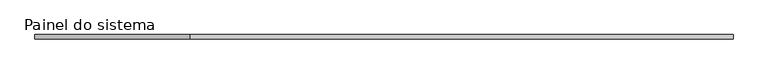
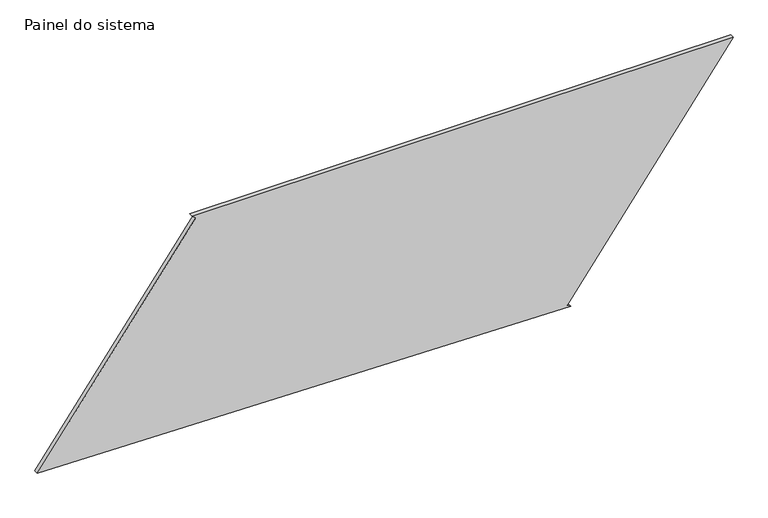
"""IFC4 building model written with IfcOpenShell, lengths in millimetres: plate geometry, Painel do sistema : Envidraçado."""

from ifc_helpers import new_model, si_unit, frame, origin, place, context, project, spatial, polyline, outline, extrude, source, transform, mapped, element, save


def painel_do_sistema_9dc0dc6b(model_context):
    return source(origin(), model_context, "Body", "SweptSolid", [
        extrude(outline(polyline([(0.0, 1085.2779269), (14.8374505, 1065.1570406), (1331.9769726, 2036.4359499), (1331.9769726, -1128.9675364), (1317.1395221, -1108.8466501), (59.2469484, -2036.4359499), (0.0, 1085.2779269)])), frame((0.0, 24.5, 0.0), z_axis=(0.0, 1.0, 0.0), x_axis=(0.0, 0.0, 1.0)), (0.0, 0.0, 1.0), 25.0),
    ])


if __name__ == "__main__":
    model = new_model("IFC4")
    model_context = context("Model", 3, world=origin())
    ifc_project = project(units=[si_unit("LENGTHUNIT", "METRE", prefix="MILLI")], contexts=[model_context])
    site = spatial("IfcSite", under=ifc_project)
    building = spatial("IfcBuilding", under=site)
    placement = place(None, origin())
    painel_do_sistema_shape = painel_do_sistema_9dc0dc6b(model_context)
    element("IfcPlate", 1, ObjectType="Painel do sistema : Envidraçado", at=placement, inside=building, context=model_context, shape_type="MappedRepresentation", body=[
        mapped(painel_do_sistema_shape, transform((0.0, 0.0, 0.0), x_axis=(1.0, 0.0, 0.0), y_axis=(0.0, 1.0, 0.0), z_axis=(0.0, 0.0, 1.0))),
    ])
    save(model, "model.ifc")

# Revit data of these elements
# Type "Painel do sistema : Envidraçado"
#   Construction Type Id = "GSP4R"
#   Analytic Construction = "Vidraça única Pilkington 1/8 pol"
#   Visual Light Transmittance = 0.9
#   Solar Heat Gain Coefficient = 0.86
#   Heat Transfer Coefficient (U) = 6.7069 W/(m²·K)
# Element 1 (IfcPlate, "Painel do sistema : Envidraçado")
#   Materials on its faces: "Vidro"
# Materials
#   "Vidro": class "Vidro", colour RGB 0 128 192, transparency 0.9, Description = "Vidro de sílica", Cost = 0
